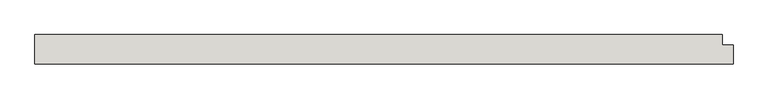
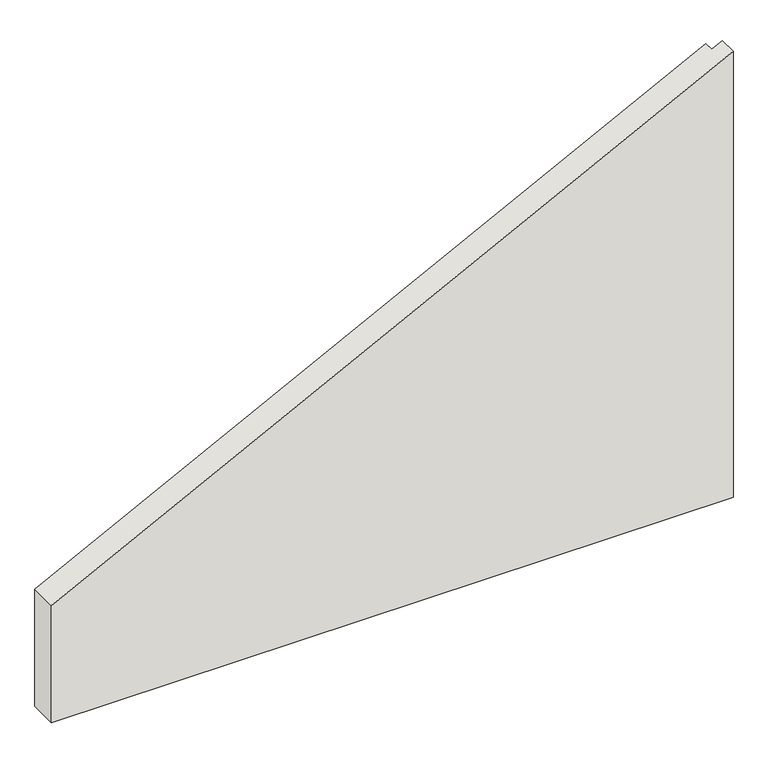
"""IFC4 building model written with IfcOpenShell, lengths in millimetres: wall geometry, Holzwand."""

from ifc_helpers import new_model, si_unit, origin, place, context, project, spatial, faceted_brep, source, transform, mapped, element, save


def wall_43baf2c4(model_context):
    return source(origin(), model_context, "Body", "Brep", [
        faceted_brep([(0.0, 200.0, 863.3339073), (0.0, 0.0, 863.3339073), (4750.0, 0.0, 3283.5797924), (4750.0, 130.0, 3283.5797924), (4675.0, 130.0, 3245.3653837), (4675.0, 200.0, 3245.3653837), (4750.0, 130.0, 0.0), (4675.0, 130.0, 0.0), (0.0, 0.0, 0.0), (4750.0, 0.0, 0.0), (0.0, 200.0, 0.0), (4675.0, 200.0, 0.0)], [[[0, 1, 2, 3, 4, 5]], [[4, 3, 6, 7]], [[2, 1, 8, 9]], [[1, 0, 10, 8]], [[0, 5, 11, 10]], [[5, 4, 7, 11]], [[9, 6, 3, 2]], [[9, 8, 10, 11, 7, 6]]]),
    ])


if __name__ == "__main__":
    model = new_model("IFC4")
    model_context = context("Model", 3, world=origin())
    ifc_project = project(units=[si_unit("LENGTHUNIT", "METRE", prefix="MILLI")], contexts=[model_context])
    site = spatial("IfcSite", under=ifc_project)
    building = spatial("IfcBuilding", under=site)
    placement = place(None, origin())
    wall_shape = wall_43baf2c4(model_context)
    element("IfcWall", 1, ObjectType="Holzwand", at=placement, inside=building, context=model_context, shape_type="MappedRepresentation", body=[
        mapped(wall_shape, transform((0.0, 0.0, 0.0), x_axis=(1.0, 0.0, 0.0), y_axis=(0.0, 1.0, 0.0), z_axis=(0.0, 0.0, 1.0))),
    ])
    save(model, "model.ifc")

# Revit data of these elements
# Element 1 (IfcWall, "Holzwand")
#   Materials on its faces: "holzschalung"
# Materials
#   "holzschalung": class "Unassigned", colour RGB 128 128 128, transparency 0
